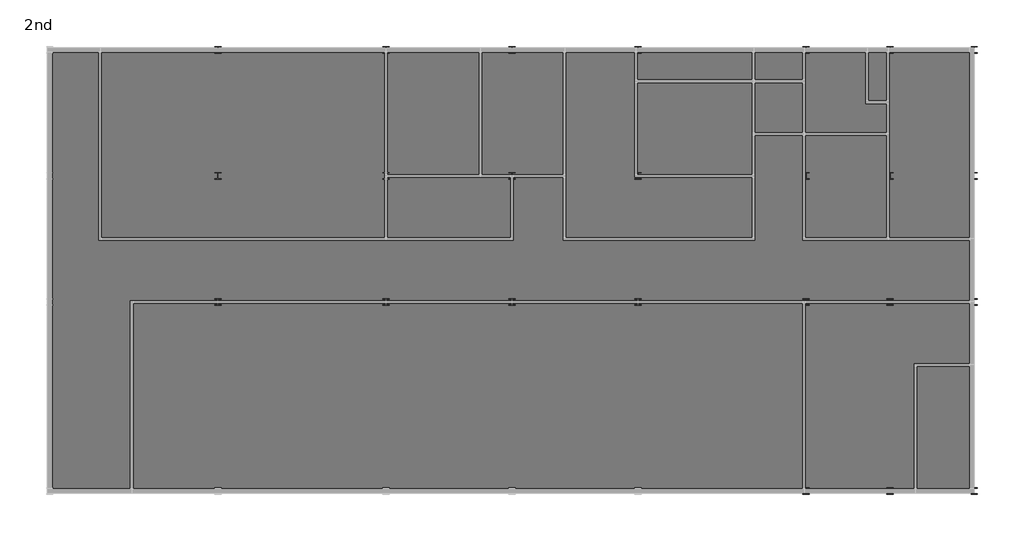
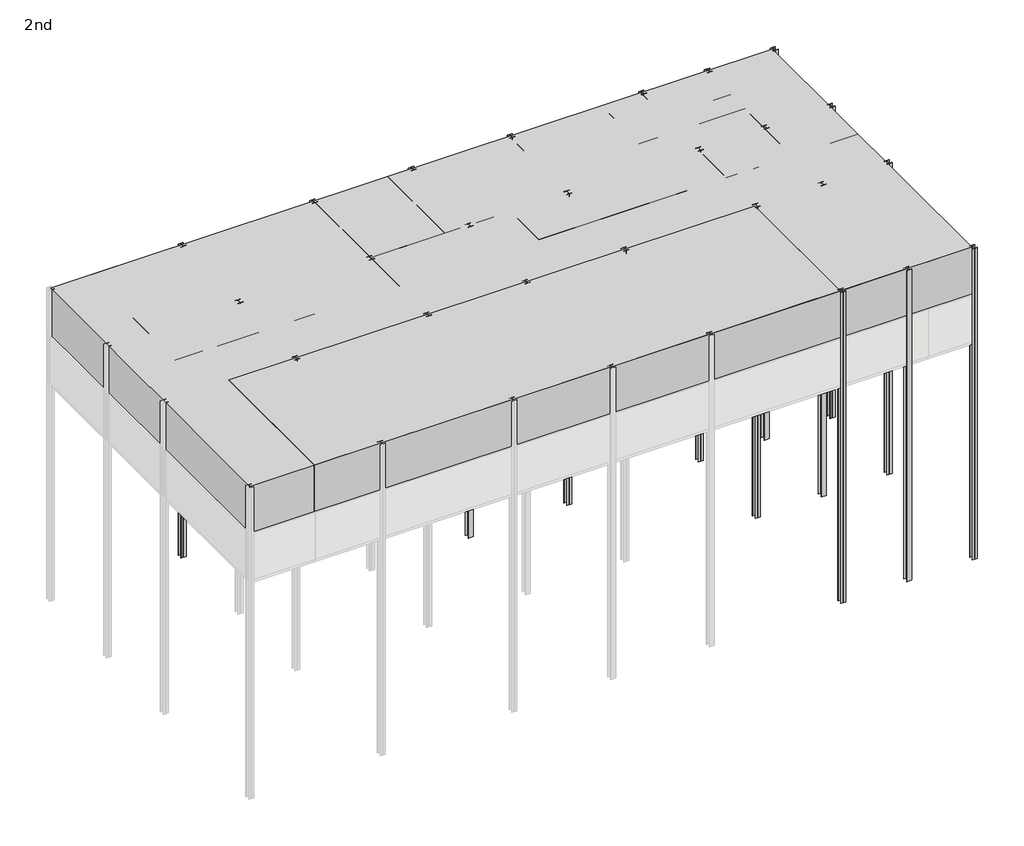
# One storey, part 3 of 3: 18 columns, 17 proxies.
# Revit data of these elements (continued)
# Element 6 (IfcBuildingElementProxy, "Space Planning Box_hec : Space Planning Box_hec") (continued)
#   Materials on its faces: "Lavender"
# Element 7 (IfcBuildingElementProxy, "Space Planning Box_hec : Space Planning Box_hec")
#   Room Name = "Locker Room (F)"
#   Interior Finish = "IF2-1"
#   Exterior Finish = "EF1"
#   Department = "AR"
#   Width = 2400 mm
#   Program Area = 31.5 m²
#   Length = 4000 mm
#   Height = 6000 mm
#   Area = 9.6 m²
#   Fill Color = Lavender
#   Phase Created = New Construction
#   Materials on its faces: "Lavender"
# Element 8 (IfcBuildingElementProxy, "Space Planning Box_hec : Space Planning Box_hec")
#   Room Name = "Shower Room (F)"
#   Interior Finish = "IF5"
#   Exterior Finish = "EF1"
#   Department = "AR"
#   Width = 2400 mm
#   Program Area = 31.5 m²
#   Length = 1500 mm
#   Height = 6000 mm
#   Area = 3.6 m²
#   Fill Color = Lavender
#   Phase Created = New Construction
#   Materials on its faces: "Lavender"
# Element 9 (IfcBuildingElementProxy, "Space Planning Box_hec : Space Planning Box_hec")
#   Room Name = "Locker Room (M)"
#   Interior Finish = "IF2-1"
#   Exterior Finish = "EF1"
#   Department = "AR"
#   Width = 5600 mm
#   Program Area = 31.5 m²
#   Length = 6000 mm
#   Height = 6000 mm
#   Area = 33.6 m²
#   Fill Color = Lavender
#   Phase Created = New Construction
#   Materials on its faces: "Lavender"
# Element 10 (IfcBuildingElementProxy, "Space Planning Box_hec : Space Planning Box_hec")
#   Room Name = "Shower Room (M)"
#   Interior Finish = "IF5"
#   Exterior Finish = "EF1"
#   Department = "AR"
#   Width = 5600 mm
#   Program Area = 31.5 m²
#   Length = 1500 mm
#   Height = 6000 mm
#   Area = 8.4 m²
#   Fill Color = Lavender
#   Phase Created = New Construction
#   Materials on its faces: "Lavender"
# Element 11 (IfcBuildingElementProxy, "Space Planning Box_hec : Space Planning Box_hec")
#   Room Name = "Kitch & Lunch Room"
#   Interior Finish = "IF2-1"
#   Exterior Finish = "EF1"
#   Department = "AR"
#   Width = 9000 mm
#   Program Area = 31.5 m²
#   Length = 9000 mm
#   Height = 6000 mm
#   Area = 81 m²
#   Fill Color = Lavender
#   Phase Created = New Construction
#   Materials on its faces: "Lavender"
# Element 12 (IfcBuildingElementProxy, "Space Planning Box_hec : Space Planning Box_hec")
#   Room Name = "Shift Office Room"
#   Interior Finish = "IF2-1"
#   Exterior Finish = "EF1"
#   Department = "AR"
#   Width = 4000 mm
#   Program Area = 43.2 m²
#   Length = 6000 mm
#   Height = 6000 mm
#   Area = 24 m²
#   Fill Color = Lavender
#   Phase Created = New Construction
#   Materials on its faces: "Lavender"
# Element 13 (IfcBuildingElementProxy, "Space Planning Box_hec : Space Planning Box_hec")
#   Room Name = "Document Room"
#   Interior Finish = "IF2-1"
#   Exterior Finish = "EF1"
#   Department = "AR"
#   Width = 4500 mm
#   Program Area = 48 m²
#   Length = 6000 mm
#   Height = 6000 mm
#   Area = 27 m²
#   Fill Color = Lavender
#   Phase Created = New Construction
#   Materials on its faces: "Lavender"
# Element 14 (IfcBuildingElementProxy, "Space Planning Box_hec : Space Planning Box_hec")
#   Room Name = "LOTO Office Room"
#   Interior Finish = "IF2-1"
#   Exterior Finish = "EF1"
#   Department = "AR"
#   Width = 3000 mm
#   Program Area = 31.5 m²
#   Length = 6000 mm
#   Height = 6000 mm
#   Area = 18 m²
#   Fill Color = Lavender
#   Phase Created = New Construction
#   Materials on its faces: "Lavender"
# Element 15 (IfcBuildingElementProxy, "Space Planning Box_hec : Space Planning Box_hec")
#   Room Name = "Engineer Room"
#   Interior Finish = "IF3"
#   Exterior Finish = "EF1"
#   Department = "CI"
#   Width = 9000 mm
#   Program Area = 120 m²
#   Length = 13600 mm
#   Height = 6000 mm
#   Area = 122.4 m²
#   Fill Color = Lime
#   Phase Created = New Construction
#   Materials on its faces: "Lime"
# Element 16 (IfcBuildingElementProxy, "Space Planning Box_hec : Space Planning Box_hec")
#   Room Name = "Fire Gas Room"
#   Interior Finish = "IF1"
#   Exterior Finish = "EF1"
#   Department = "SF"
#   Width = 8000 mm
#   Program Area = 0 m²
#   Length = 9000 mm
#   Height = 6000 mm
#   Area = 72 m²
#   Fill Color = Cyan
#   Phase Created = New Construction
#   Materials on its faces: "Cyan"
# Element 17 (IfcBuildingElementProxy, "Space Planning Box_hec : Space Planning Box_hec")
#   Room Name = "Corridor"
#   Interior Finish = "IF2-1"
#   Exterior Finish = "EF1"
#   Department = "AR"
#   Width = 43900 mm
#   Program Area = 0 m²
#   Length = 21000 mm
#   Height = 6000 mm
#   Area = 921.9 m²
#   Fill Color = Lavender
#   Phase Created = New Construction
#   Materials on its faces: "Lavender"
# Elements 18, 19, 20, 21, 22, 23, 24, 25, 26, 27, 28, 29, 30, 31, 32, 33, 34, 35 (IfcColumn, "UC-Universal Columns-Column : UC305x305x97")
#   Structural Material = Metal - Steel 43-275
#   Phase Created = New Construction
#   Materials on its faces: "Metal - Steel 43-275"
# Materials
#   "Cyan": class "Generic", colour RGB 0 255 255, transparency 0.2, Cost = 0
#   "Metal - Steel 43-275": class "Metal", colour RGB 247 247 247, transparency 0, Cost = 0
#   "Lavender": class "Generic", colour RGB 186 85 211, transparency 0.2, Cost = 0
#   "Pink": class "Generic", colour RGB 255 105 180, transparency 0.2, Cost = 0
#   "Lime": class "Generic", colour RGB 0 255 0, transparency 0.2, Cost = 0
